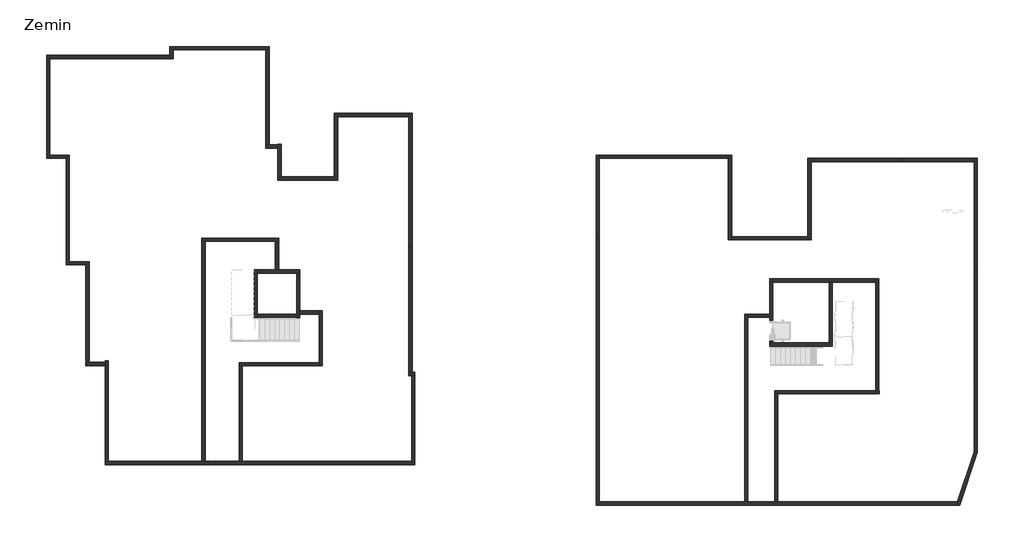
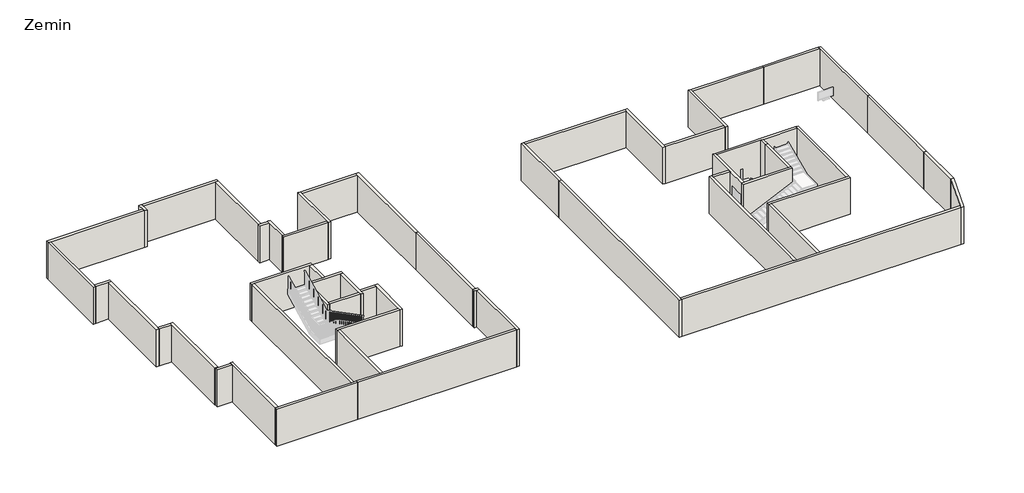
# One storey, part 1 of 2: 56 walls.
"""IFC4 building model written with IfcOpenShell, lengths in millimetres."""

from ifc_helpers import new_model, si_unit, origin, origin_with_axes, place, context, project, spatial, polyline, outline, extrude, faceted_brep, element, save

model = new_model("IFC4")

# Units and contexts
model_context = context("Model", 3, world=origin())
ifc_project = project(units=[si_unit("LENGTHUNIT", "METRE", prefix="MILLI")], contexts=[model_context])

# Site, building, storey
site = spatial("IfcSite", under=ifc_project)
building = spatial("IfcBuilding", under=site)
storey = spatial("IfcBuildingStorey", under=building, Name="Zemin", Elevation=0.0)

# Walls
placement = place(None, origin())
element("IfcWall", 1, ObjectType="Generic - 200mm", at=placement, inside=storey, context=model_context, shape_type="Brep", body=[
    faceted_brep([(25749.836337, 7619.475628, 0.0), (30068.3425199, 7619.475628, 0.0), (30068.3425199, 7619.475628, 3000.0), (25749.836337, 7619.475628, 3000.0), (25749.836337, 7819.475628, 0.0), (25749.836337, 7819.475628, 3000.0), (30068.3425199, 7819.475628, 3000.0), (30068.3425199, 7819.475628, 0.0), (30068.3425199, 7621.2707349, 3000.0)], [[[0, 1, 2, 3]], [[4, 5, 6, 7]], [[1, 0, 4, 7]], [[3, 2, 8, 6, 5]], [[0, 3, 5, 4]], [[2, 1, 7, 6, 8]]]),
])
element("IfcWall", 2, ObjectType="Generic - 200mm", at=placement, inside=storey, context=model_context, shape_type="Brep", body=[
    faceted_brep([(30068.3425199, 7819.475628, 0.0), (30068.3425199, 7619.475628, 0.0), (30068.3425199, 1319.475628, 0.0), (30068.3425199, 1319.475628, 3000.0), (30068.3425199, 7619.475628, 3000.0), (30068.3425199, 7819.475628, 3000.0), (30268.3425199, 7819.475628, 0.0), (30268.3425199, 7819.475628, 3000.0), (30268.3425199, 1319.475628, 3000.0), (30268.3425199, 1319.475628, 0.0), (30068.8612349, 1319.475628, 0.0), (30068.8612349, 1319.475628, 3000.0)], [[[0, 1, 2, 3, 4, 5]], [[6, 7, 8, 9]], [[2, 1, 0, 6, 9, 10]], [[3, 2, 10, 9, 8, 11]], [[5, 4, 3, 11, 8, 7]], [[0, 5, 7, 6]]]),
])
element("IfcWall", 3, ObjectType="Generic - 200mm", at=placement, inside=storey, context=model_context, shape_type="Brep", body=[
    faceted_brep([(30068.8612349, 1319.475628, 0.0), (30068.8612349, -6240.0098119, 0.0), (30068.8612349, -6240.0098119, 3000.0), (30068.8612349, 1319.475628, 3000.0), (30268.8612349, 1319.475628, 0.0), (30268.8612349, 1319.475628, 3000.0), (30268.8612349, -6240.0098119, 3000.0), (30268.8612349, -6240.0098119, 0.0), (30268.3425199, 1319.475628, 0.0), (30069.3799498, -6240.0098119, 0.0), (30069.3799498, -6240.0098119, 3000.0), (30268.3425199, 1319.475628, 3000.0)], [[[0, 1, 2, 3]], [[4, 5, 6, 7]], [[1, 0, 8, 4, 7, 9]], [[2, 1, 9, 7, 6, 10]], [[3, 2, 10, 6, 5, 11]], [[0, 3, 11, 5, 4, 8]]]),
])
element("IfcWall", 4, ObjectType="Generic - 200mm", at=placement, inside=storey, context=model_context, shape_type="Brep", body=[
    faceted_brep([(30069.3799498, -6240.0098119, 0.0), (30069.3799498, -9831.8731192, 0.0), (30069.3799498, -9831.8731192, 3000.0), (30069.3799498, -9830.0780123, 3000.0), (30069.3799498, -6240.0098119, 3000.0), (30269.3799498, -6240.0098119, 0.0), (30269.3799498, -6240.0098119, 3000.0), (30269.3799498, -9862.9162623, 3000.0), (30269.3799498, -9864.7113693, 3000.0), (30269.3799498, -9864.7113693, 0.0), (30268.8612349, -6240.0098119, 0.0), (30268.8612349, -6240.0098119, 3000.0)], [[[0, 1, 2, 3, 4]], [[5, 6, 7, 8, 9]], [[1, 0, 10, 5, 9]], [[4, 3, 2, 8, 7, 6, 11]], [[0, 4, 11, 6, 5, 10]], [[2, 1, 9, 8]]]),
])
element("IfcWall", 5, ObjectType="Generic - 200mm", at=placement, inside=storey, context=model_context, shape_type="Brep", body=[
    faceted_brep([(21549.836337, -3276.2808257, 0.0), (21349.836337, -3276.2808257, 0.0), (17970.6041014, -3276.2808257, 0.0), (17770.6041014, -3276.2808257, 0.0), (17770.6041014, -3276.2808257, 3000.0), (17970.6041014, -3276.2808257, 3000.0), (21349.836337, -3276.2808257, 3000.0), (21549.836337, -3276.2808257, 3000.0), (21549.836337, -3476.2808257, 0.0), (21549.836337, -3476.2808257, 3000.0), (17770.6041014, -3476.2808257, 3000.0), (17770.6041014, -3476.2808257, 0.0), (17770.6041014, -3474.4857187, 3000.0), (21549.836337, -3474.4857187, 3000.0)], [[[0, 1, 2, 3, 4, 5, 6, 7]], [[8, 9, 10, 11]], [[3, 2, 1, 0, 8, 11]], [[7, 6, 5, 4, 12, 10, 9, 13]], [[0, 7, 13, 9, 8]], [[4, 3, 11, 10, 12]]]),
])
element("IfcWall", 6, ObjectType="Generic - 200mm", at=placement, inside=storey, context=model_context, shape_type="Brep", body=[
    faceted_brep([(29055.3124022, -12836.6907835, 0.0), (18270.6041014, -12836.6907835, 0.0), (18070.6041014, -12836.6907835, 0.0), (16470.6041014, -12836.6907835, 0.0), (16270.6041014, -12836.6907835, 0.0), (7543.716007, -12836.6907835, 0.0), (7543.716007, -12836.6907835, 3000.0), (16270.6041014, -12836.6907835, 3000.0), (16470.6041014, -12836.6907835, 3000.0), (18070.6041014, -12836.6907835, 3000.0), (18270.6041014, -12836.6907835, 3000.0), (29055.3124022, -12836.6907835, 3000.0), (28987.8162902, -13036.6907835, 0.0), (28987.8162902, -13036.6907835, 3000.0), (7543.716007, -13036.6907835, 3000.0), (7543.716007, -13036.6907835, 0.0), (7543.716007, -13034.8956765, 3000.0)], [[[0, 1, 2, 3, 4, 5, 6, 7, 8, 9, 10, 11]], [[12, 13, 14, 15]], [[5, 4, 3, 2, 1, 0, 12, 15]], [[11, 10, 9, 8, 7, 6, 16, 14, 13]], [[0, 11, 13, 12]], [[6, 5, 15, 14, 16]]]),
])
element("IfcWall", 7, ObjectType="Generic - 200mm", at=placement, inside=storey, context=model_context, shape_type="Brep", body=[
    faceted_brep([(30069.3799498, -9831.8731192, 0.0), (29055.3124022, -12836.6907835, 0.0), (28987.8162902, -13036.6907835, 0.0), (28987.8162902, -13036.6907835, 3000.0), (29055.3124022, -12836.6907835, 3000.0), (30069.3799498, -9831.8731192, 3000.0), (30269.3799498, -9864.7113693, 0.0), (30269.3799498, -9864.7113693, 3000.0), (29198.8985612, -13036.6907835, 3000.0), (29198.8985612, -13036.6907835, 0.0)], [[[0, 1, 2, 3, 4, 5]], [[6, 7, 8, 9]], [[2, 1, 0, 6, 9]], [[5, 4, 3, 8, 7]], [[0, 5, 7, 6]], [[3, 2, 9, 8]]]),
])
element("IfcWall", 8, ObjectType="Generic - 200mm", at=placement, inside=storey, context=model_context, shape_type="Brep", body=[
    faceted_brep([(24363.3998354, -6140.0098119, 0.0), (24348.8612349, -6140.0098119, 0.0), (24148.8612349, -6140.0098119, 0.0), (18070.6041014, -6140.0098119, 0.0), (18070.6041014, -6140.0098119, 3000.0), (24148.8612349, -6140.0098119, 3000.0), (24348.8612349, -6140.0098119, 3000.0), (24363.3998354, -6140.0098119, 3000.0), (24363.3998354, -6340.0098119, 0.0), (24363.3998354, -6340.0098119, 3000.0), (18270.6041014, -6340.0098119, 3000.0), (18070.6041014, -6340.0098119, 3000.0), (18070.6041014, -6340.0098119, 0.0), (18270.6041014, -6340.0098119, 0.0)], [[[0, 1, 2, 3, 4, 5, 6, 7]], [[8, 9, 10, 11, 12, 13]], [[3, 2, 1, 0, 8, 13, 12]], [[7, 6, 5, 4, 11, 10, 9]], [[0, 7, 9, 8]], [[4, 3, 12, 11]]]),
])
element("IfcWall", 9, ObjectType="Generic - 200mm", at=placement, inside=storey, context=model_context, shape_type="Brep", body=[
    faceted_brep([(7343.716007, 3020.535295, 0.0), (7343.716007, -13036.6907835, 0.0), (7343.716007, -13036.6907835, 3000.0), (7343.716007, -13034.8956765, 3000.0), (7343.716007, 2920.535295, 3000.0), (7343.716007, 3020.535295, 3000.0), (7543.716007, 3020.535295, 0.0), (7543.716007, 3020.535295, 3000.0), (7543.716007, 2920.535295, 3000.0), (7543.716007, -12836.6907835, 3000.0), (7543.716007, -13034.8956765, 3000.0), (7543.716007, -13036.6907835, 3000.0), (7543.716007, -13036.6907835, 0.0), (7543.716007, -12836.6907835, 0.0)], [[[0, 1, 2, 3, 4, 5]], [[6, 7, 8, 9, 10, 11, 12, 13]], [[1, 0, 6, 13, 12]], [[5, 4, 3, 2, 11, 10, 9, 8, 7]], [[0, 5, 7, 6]], [[2, 1, 12, 11]]]),
])
element("IfcWall", 10, ObjectType="Generic - 200mm", at=placement, inside=storey, context=model_context, shape_type="Brep", body=[
    faceted_brep([(24348.8612349, -6140.0098119, 0.0), (24348.8612349, 579.475628, 0.0), (24348.8612349, 579.475628, 3000.0), (24348.8612349, -6140.0098119, 3000.0), (24148.8612349, -6140.0098119, 0.0), (24148.8612349, -6140.0098119, 3000.0), (24148.8612349, 379.475628, 3000.0), (24148.8612349, 579.475628, 3000.0), (24148.8612349, 579.475628, 0.0), (24148.8612349, 379.475628, 0.0)], [[[0, 1, 2, 3]], [[4, 5, 6, 7, 8, 9]], [[1, 0, 4, 9, 8]], [[3, 2, 7, 6, 5]], [[0, 3, 5, 4]], [[2, 1, 8, 7]]]),
])
element("IfcWall", 11, ObjectType="Generic - 200mm", at=placement, inside=storey, context=model_context, shape_type="Brep", body=[
    faceted_brep([(21349.836337, -200.524372, 0.0), (21349.836337, -3276.2808257, 0.0), (21349.836337, -3276.2808257, 3000.0), (21349.836337, -3274.4857187, 3000.0), (21349.836337, -200.524372, 3000.0), (21549.836337, -200.524372, 0.0), (21549.836337, -200.524372, 3000.0), (21549.836337, -3274.4857187, 3000.0), (21549.836337, -3276.2808257, 3000.0), (21549.836337, -3276.2808257, 0.0)], [[[0, 1, 2, 3, 4]], [[5, 6, 7, 8, 9]], [[1, 0, 5, 9]], [[4, 3, 2, 8, 7, 6]], [[0, 4, 6, 5]], [[2, 1, 9, 8]]]),
])
element("IfcWall", 12, ObjectType="Generic - 200mm", at=placement, inside=storey, context=model_context, shape_type="Brep", body=[
    faceted_brep([(17770.6041014, -3276.2808257, 3000.0), (17770.6041014, -3274.4857187, 3000.0), (17770.6041014, -3179.4925158, 3000.0), (17770.6041014, -1924.4857188, 3000.0), (17770.6041014, -1740.0098119, 3000.0), (17770.6041014, -1540.0098119, 3000.0), (17770.6041014, 579.475628, 3000.0), (17770.6041014, 579.475628, 0.0), (17770.6041014, -1540.0098119, 0.0), (17770.6041014, -1740.0098119, 0.0), (17770.6041014, -1926.2808257, 0.0), (17770.6041014, -1926.2808257, 2000.0), (17770.6041014, -3181.2876228, 2000.0), (17770.6041014, -3181.2876228, 0.0), (17770.6041014, -3276.2808257, 0.0), (17970.6041014, 579.475628, 3000.0), (17970.6041014, 379.475628, 3000.0), (17970.6041014, -1924.4857188, 3000.0), (17970.6041014, -3179.4925158, 3000.0), (17970.6041014, -3274.4857187, 3000.0), (17970.6041014, -3276.2808257, 3000.0), (17970.6041014, -3276.2808257, 0.0), (17970.6041014, -3181.2876228, 0.0), (17970.6041014, -3181.2876228, 2000.0), (17970.6041014, -1926.2808257, 2000.0), (17970.6041014, -1926.2808257, 0.0), (17970.6041014, 379.475628, 0.0), (17970.6041014, 579.475628, 0.0)], [[[0, 1, 2, 3, 4, 5, 6, 7, 8, 9, 10, 11, 12, 13, 14]], [[15, 16, 17, 18, 19, 20, 21, 22, 23, 24, 25, 26, 27]], [[21, 14, 13, 22]], [[7, 27, 26, 25, 10, 9, 8]], [[6, 5, 4, 3, 2, 1, 0, 20, 19, 18, 17, 16, 15]], [[0, 14, 21, 20]], [[12, 23, 22, 13]], [[24, 11, 10, 25]], [[11, 24, 23, 12]], [[27, 7, 6, 15]]]),
])
element("IfcWall", 13, ObjectType="Generic - 200mm", at=placement, inside=storey, context=model_context, shape_type="SweptSolid", body=[
    extrude(outline(polyline([(21549.836337, 379.475628), (21549.836337, -200.524372), (21349.836337, -200.524372), (21349.836337, 379.475628), (21549.836337, 379.475628)])), origin_with_axes(), (0.0, 0.0, 1.0), 3000.0),
])
element("IfcWall", 14, ObjectType="Generic - 200mm", at=placement, inside=storey, context=model_context, shape_type="Brep", body=[
    faceted_brep([(20268.8612349, 7619.475628, 0.0), (25749.836337, 7619.475628, 0.0), (25749.836337, 7619.475628, 3000.0), (20268.8612349, 7619.475628, 3000.0), (20268.8612349, 7819.475628, 0.0), (20268.8612349, 7819.475628, 3000.0), (25749.836337, 7819.475628, 3000.0), (25749.836337, 7819.475628, 0.0), (20268.8612349, 7621.2707349, 3000.0)], [[[0, 1, 2, 3]], [[4, 5, 6, 7]], [[1, 0, 4, 7]], [[2, 1, 7, 6]], [[3, 2, 6, 5, 8]], [[0, 3, 8, 5, 4]]]),
])
element("IfcWall", 15, ObjectType="Generic - 200mm", at=placement, inside=storey, context=model_context, shape_type="Brep", body=[
    faceted_brep([(16470.6041014, -12836.6907835, 0.0), (16470.6041014, -1740.0098119, 0.0), (16470.6041014, -1540.0098119, 0.0), (16470.6041014, -1540.0098119, 3000.0), (16470.6041014, -1740.0098119, 3000.0), (16470.6041014, -12836.6907835, 3000.0), (16270.6041014, -12836.6907835, 0.0), (16270.6041014, -12836.6907835, 3000.0), (16270.6041014, -1540.0098119, 3000.0), (16270.6041014, -1540.0098119, 0.0)], [[[0, 1, 2, 3, 4, 5]], [[6, 7, 8, 9]], [[2, 1, 0, 6, 9]], [[5, 4, 3, 8, 7]], [[3, 2, 9, 8]], [[0, 5, 7, 6]]]),
])
element("IfcWall", 16, ObjectType="Generic - 200mm", at=placement, inside=storey, context=model_context, shape_type="Brep", body=[
    faceted_brep([(20068.8612349, 7819.475628, 0.0), (20068.8612349, 3119.475628, 0.0), (20068.8612349, 2919.475628, 0.0), (20068.8612349, 2919.475628, 3000.0), (20068.8612349, 2921.2707349, 3000.0), (20068.8612349, 3119.475628, 3000.0), (20068.8612349, 7819.475628, 3000.0), (20268.8612349, 7819.475628, 0.0), (20268.8612349, 7819.475628, 3000.0), (20268.8612349, 7619.475628, 3000.0), (20268.8612349, 2921.2707349, 3000.0), (20268.8612349, 2919.475628, 3000.0), (20268.8612349, 2919.475628, 0.0), (20268.8612349, 7619.475628, 0.0)], [[[0, 1, 2, 3, 4, 5, 6]], [[7, 8, 9, 10, 11, 12, 13]], [[2, 1, 0, 7, 13, 12]], [[6, 5, 4, 3, 11, 10, 9, 8]], [[0, 6, 8, 7]], [[3, 2, 12, 11]]]),
])
element("IfcWall", 17, ObjectType="Generic - 200mm", at=placement, inside=storey, context=model_context, shape_type="Brep", body=[
    faceted_brep([(24148.8612349, 579.475628, 0.0), (17970.6041014, 579.475628, 0.0), (17970.6041014, 579.475628, 3000.0), (24148.8612349, 579.475628, 3000.0), (24148.8612349, 379.475628, 0.0), (24148.8612349, 379.475628, 3000.0), (21549.836337, 379.475628, 3000.0), (21349.836337, 379.475628, 3000.0), (17970.6041014, 379.475628, 3000.0), (17970.6041014, 379.475628, 0.0), (21349.836337, 379.475628, 0.0), (21549.836337, 379.475628, 0.0)], [[[0, 1, 2, 3]], [[4, 5, 6, 7, 8, 9, 10, 11]], [[1, 0, 4, 11, 10, 9]], [[3, 2, 8, 7, 6, 5]], [[2, 1, 9, 8]], [[0, 3, 5, 4]]]),
])
element("IfcWall", 18, ObjectType="Generic - 200mm", at=placement, inside=storey, context=model_context, shape_type="Brep", body=[
    faceted_brep([(-3749.8304233, -5256.848891, 0.0), (-3749.8304233, -10389.1627129, 0.0), (-3749.8304233, -10589.1627129, 0.0), (-3749.8304233, -10589.1627129, 3000.0), (-3749.8304233, -10587.367606, 3000.0), (-3749.8304233, -10389.1627129, 3000.0), (-3749.8304233, -5256.848891, 3000.0), (-3549.8304233, -5256.848891, 0.0), (-3549.8304233, -5256.848891, 3000.0), (-3549.8304233, -10587.367606, 3000.0), (-3549.8304233, -10589.1627129, 3000.0), (-3549.8304233, -10589.1627129, 0.0)], [[[0, 1, 2, 3, 4, 5, 6]], [[7, 8, 9, 10, 11]], [[2, 1, 0, 7, 11]], [[6, 5, 4, 3, 10, 9, 8]], [[3, 2, 11, 10]], [[0, 6, 8, 7]]]),
])
element("IfcWall", 19, ObjectType="Generic - 200mm", at=placement, inside=storey, context=model_context, shape_type="Brep", body=[
    faceted_brep([(-3749.8304233, -10389.1627129, 0.0), (-13926.101437, -10389.1627129, 0.0), (-14126.101437, -10389.1627129, 0.0), (-15974.8304233, -10389.1627129, 0.0), (-15974.8304233, -10389.1627129, 3000.0), (-14126.101437, -10389.1627129, 3000.0), (-13926.101437, -10389.1627129, 3000.0), (-3749.8304233, -10389.1627129, 3000.0), (-3749.8304233, -10589.1627129, 0.0), (-3749.8304233, -10589.1627129, 3000.0), (-15974.8304233, -10589.1627129, 3000.0), (-15974.8304233, -10589.1627129, 0.0), (-15974.8304233, -10389.6814279, 0.0), (-15974.8304233, -10587.367606, 3000.0), (-15974.8304233, -10389.6814279, 3000.0), (-3749.8304233, -10587.367606, 3000.0)], [[[0, 1, 2, 3, 4, 5, 6, 7]], [[8, 9, 10, 11]], [[3, 2, 1, 0, 8, 11, 12]], [[4, 3, 12, 11, 10, 13, 14]], [[7, 6, 5, 4, 14, 13, 10, 9, 15]], [[0, 7, 15, 9, 8]]]),
])
element("IfcWall", 20, ObjectType="Generic - 200mm", at=placement, inside=storey, context=model_context, shape_type="Brep", body=[
    faceted_brep([(-15974.8304233, -10389.6814279, 0.0), (-16173.9741722, -10389.6814279, 0.0), (-16373.9741722, -10389.6814279, 0.0), (-21985.6447259, -10389.6814279, 0.0), (-22185.6447259, -10389.6814279, 0.0), (-22185.6447259, -10389.6814279, 3000.0), (-21985.6447259, -10389.6814279, 3000.0), (-16373.9741722, -10389.6814279, 3000.0), (-16173.9741722, -10389.6814279, 3000.0), (-15974.8304233, -10389.6814279, 3000.0), (-15974.8304233, -10589.6814279, 0.0), (-15974.8304233, -10589.6814279, 3000.0), (-22185.6447259, -10589.6814279, 3000.0), (-22185.6447259, -10589.6814279, 0.0), (-15974.8304233, -10589.1627129, 0.0), (-22185.6447259, -10587.886321, 3000.0), (-15974.8304233, -10589.1627129, 3000.0), (-15974.8304233, -10587.886321, 3000.0)], [[[0, 1, 2, 3, 4, 5, 6, 7, 8, 9]], [[10, 11, 12, 13]], [[4, 3, 2, 1, 0, 14, 10, 13]], [[9, 8, 7, 6, 5, 15, 12, 11, 16, 17]], [[0, 9, 17, 16, 11, 10, 14]], [[5, 4, 13, 12, 15]]]),
])
element("IfcWall", 21, ObjectType="Generic - 200mm", at=placement, inside=storey, context=model_context, shape_type="Brep", body=[
    faceted_brep([(-13026.101437, -1740.1378151, 0.0), (-13026.101437, -1540.1378151, 0.0), (-13026.101437, 920.8372871, 0.0), (-13026.101437, 1120.8372871, 0.0), (-13026.101437, 1120.8372871, 3000.0), (-13026.101437, 920.8372871, 3000.0), (-13026.101437, -1540.1378151, 3000.0), (-13026.101437, -1738.3427081, 3000.0), (-13026.101437, -1740.1378151, 3000.0), (-13226.101437, -1740.1378151, 0.0), (-13226.101437, -1740.1378151, 3000.0), (-13226.101437, -1738.3427081, 3000.0), (-13226.101437, 1120.8372871, 3000.0), (-13226.101437, 1120.8372871, 0.0)], [[[0, 1, 2, 3, 4, 5, 6, 7, 8]], [[9, 10, 11, 12, 13]], [[3, 2, 1, 0, 9, 13]], [[8, 7, 6, 5, 4, 12, 11, 10]], [[0, 8, 10, 9]], [[4, 3, 13, 12]]]),
])
element("IfcWall", 22, ObjectType="Generic - 200mm", at=placement, inside=storey, context=model_context, shape_type="Brep", body=[
    faceted_brep([(-23146.5113948, -4345.3648645, 0.0), (-23146.5113948, 1614.6351355, 0.0), (-23146.5113948, 1614.6351355, 3000.0), (-23146.5113948, -4345.3648645, 3000.0), (-23346.5113948, -4345.3648645, 0.0), (-23346.5113948, -4345.3648645, 3000.0), (-23346.5113948, 1414.6351355, 3000.0), (-23346.5113948, 1614.6351355, 3000.0), (-23346.5113948, 1614.6351355, 0.0), (-23346.5113948, 1414.6351355, 0.0)], [[[0, 1, 2, 3]], [[4, 5, 6, 7, 8, 9]], [[1, 0, 4, 9, 8]], [[3, 2, 7, 6, 5]], [[0, 3, 5, 4]], [[2, 1, 8, 7]]]),
])
element("IfcWall", 23, ObjectType="Generic - 200mm", at=placement, inside=storey, context=model_context, shape_type="SweptSolid", body=[
    extrude(outline(polyline([(-16173.9741722, 2820.8372871), (-16173.9741722, -10389.6814279), (-16373.9741722, -10389.6814279), (-16373.9741722, 2820.8372871), (-16173.9741722, 2820.8372871)])), origin_with_axes(), (0.0, 0.0, 1.0), 3000.0),
])
element("IfcWall", 24, ObjectType="Generic - 200mm", at=placement, inside=storey, context=model_context, shape_type="Brep", body=[
    faceted_brep([(-14126.101437, -4659.1627129, 0.0), (-13926.101437, -4659.1627129, 0.0), (-9310.3884323, -4659.1627129, 0.0), (-9310.3884323, -4659.1627129, 3000.0), (-13926.101437, -4659.1627129, 3000.0), (-14126.101437, -4659.1627129, 3000.0), (-14126.101437, -4459.1627129, 0.0), (-14126.101437, -4459.1627129, 3000.0), (-9310.3884323, -4459.1627129, 3000.0), (-9310.3884323, -4459.1627129, 0.0), (-9310.3884323, -4657.367606, 3000.0)], [[[0, 1, 2, 3, 4, 5]], [[6, 7, 8, 9]], [[2, 1, 0, 6, 9]], [[5, 4, 3, 10, 8, 7]], [[3, 2, 9, 8, 10]], [[0, 5, 7, 6]]]),
])
element("IfcWall", 25, ObjectType="Generic - 200mm", at=placement, inside=storey, context=model_context, shape_type="Brep", body=[
    faceted_brep([(-10669.8304233, -1540.1378151, 0.0), (-13026.101437, -1540.1378151, 0.0), (-13026.101437, -1540.1378151, 3000.0), (-10669.8304233, -1540.1378151, 3000.0), (-10669.8304233, -1740.1378151, 0.0), (-10669.8304233, -1740.1378151, 3000.0), (-13026.101437, -1740.1378151, 3000.0), (-13026.101437, -1740.1378151, 0.0), (-13026.101437, -1738.3427081, 3000.0)], [[[0, 1, 2, 3]], [[4, 5, 6, 7]], [[1, 0, 4, 7]], [[3, 2, 8, 6, 5]], [[2, 1, 7, 6, 8]], [[0, 3, 5, 4]]]),
])
element("IfcWall", 26, ObjectType="Generic - 200mm", at=placement, inside=storey, context=model_context, shape_type="Brep", body=[
    faceted_brep([(-10469.8304233, 1120.8372871, 0.0), (-11746.101437, 1120.8372871, 0.0), (-11946.101437, 1120.8372871, 0.0), (-13026.101437, 1120.8372871, 0.0), (-13026.101437, 1120.8372871, 3000.0), (-11946.101437, 1120.8372871, 3000.0), (-11746.101437, 1120.8372871, 3000.0), (-10469.8304233, 1120.8372871, 3000.0), (-10469.8304233, 920.8372871, 0.0), (-10469.8304233, 920.8372871, 3000.0), (-10669.8304233, 920.8372871, 3000.0), (-13026.101437, 920.8372871, 3000.0), (-13026.101437, 920.8372871, 0.0), (-10669.8304233, 920.8372871, 0.0), (-13026.101437, 922.632394, 3000.0), (-10469.8304233, 922.632394, 3000.0)], [[[0, 1, 2, 3, 4, 5, 6, 7]], [[8, 9, 10, 11, 12, 13]], [[3, 2, 1, 0, 8, 13, 12]], [[7, 6, 5, 4, 14, 11, 10, 9, 15]], [[0, 7, 15, 9, 8]], [[4, 3, 12, 11, 14]]]),
])
element("IfcWall", 27, ObjectType="Generic - 200mm", at=placement, inside=storey, context=model_context, shape_type="Brep", body=[
    faceted_brep([(-10469.8304233, -1779.1627129, 0.0), (-10469.8304233, -1540.1378151, 0.0), (-10469.8304233, -1340.1378151, 0.0), (-10469.8304233, 920.8372871, 0.0), (-10469.8304233, 920.8372871, 3000.0), (-10469.8304233, -1340.1378151, 3000.0), (-10469.8304233, -1540.1378151, 3000.0), (-10469.8304233, -1777.367606, 3000.0), (-10469.8304233, -1779.1627129, 3000.0), (-10669.8304233, -1779.1627129, 0.0), (-10669.8304233, -1779.1627129, 3000.0), (-10669.8304233, -1777.367606, 3000.0), (-10669.8304233, -1740.1378151, 3000.0), (-10669.8304233, -1540.1378151, 3000.0), (-10669.8304233, 920.8372871, 3000.0), (-10669.8304233, 920.8372871, 0.0), (-10669.8304233, -1540.1378151, 0.0), (-10669.8304233, -1740.1378151, 0.0)], [[[0, 1, 2, 3, 4, 5, 6, 7, 8]], [[9, 10, 11, 12, 13, 14, 15, 16, 17]], [[3, 2, 1, 0, 9, 17, 16, 15]], [[8, 7, 6, 5, 4, 14, 13, 12, 11, 10]], [[0, 8, 10, 9]], [[4, 3, 15, 14]]]),
])
element("IfcWall", 28, ObjectType="Generic - 200mm", at=placement, inside=storey, context=model_context, shape_type="Brep", body=[
    faceted_brep([(-12326.101437, 14540.8372871, 0.0), (-18089.8304233, 14540.8372871, 0.0), (-18089.8304233, 14540.8372871, 3000.0), (-12326.101437, 14540.8372871, 3000.0), (-12326.101437, 14340.8372871, 0.0), (-12326.101437, 14340.8372871, 3000.0), (-12526.101437, 14340.8372871, 3000.0), (-18089.8304233, 14340.8372871, 3000.0), (-18089.8304233, 14340.8372871, 0.0), (-12526.101437, 14340.8372871, 0.0), (-18089.8304233, 14342.632394, 3000.0), (-12326.101437, 14342.632394, 3000.0)], [[[0, 1, 2, 3]], [[4, 5, 6, 7, 8, 9]], [[1, 0, 4, 9, 8]], [[3, 2, 10, 7, 6, 5, 11]], [[2, 1, 8, 7, 10]], [[0, 3, 11, 5, 4]]]),
])
element("IfcWall", 29, ObjectType="Generic - 200mm", at=placement, inside=storey, context=model_context, shape_type="Brep", body=[
    faceted_brep([(-25701.4369496, 13812.8400285, 0.0), (-25701.4369496, 7812.8400285, 0.0), (-25701.4369496, 7812.8400285, 3000.0), (-25701.4369496, 7814.6351355, 3000.0), (-25701.4369496, 13812.8400285, 3000.0), (-25501.4369496, 13812.8400285, 0.0), (-25501.4369496, 13812.8400285, 3000.0), (-25501.4369496, 8012.8400285, 3000.0), (-25501.4369496, 7814.6351355, 3000.0), (-25501.4369496, 7812.8400285, 3000.0), (-25501.4369496, 7812.8400285, 0.0), (-25501.4369496, 8012.8400285, 0.0)], [[[0, 1, 2, 3, 4]], [[5, 6, 7, 8, 9, 10, 11]], [[1, 0, 5, 11, 10]], [[4, 3, 2, 9, 8, 7, 6]], [[2, 1, 10, 9]], [[0, 4, 6, 5]]]),
])
element("IfcWall", 30, ObjectType="Generic - 200mm", at=placement, inside=storey, context=model_context, shape_type="Brep", body=[
    faceted_brep([(-25501.4369496, 7812.8400285, 0.0), (-24523.9741722, 7812.8400285, 0.0), (-24323.9741722, 7812.8400285, 0.0), (-24323.9741722, 7812.8400285, 3000.0), (-24523.9741722, 7812.8400285, 3000.0), (-25501.4369496, 7812.8400285, 3000.0), (-25501.4369496, 8012.8400285, 0.0), (-25501.4369496, 8012.8400285, 3000.0), (-24323.9741722, 8012.8400285, 3000.0), (-24323.9741722, 8012.8400285, 0.0), (-25501.4369496, 7814.6351355, 3000.0)], [[[0, 1, 2, 3, 4, 5]], [[6, 7, 8, 9]], [[2, 1, 0, 6, 9]], [[5, 4, 3, 8, 7, 10]], [[0, 5, 10, 7, 6]], [[3, 2, 9, 8]]]),
])
element("IfcWall", 31, ObjectType="Generic - 200mm", at=placement, inside=storey, context=model_context, shape_type="Brep", body=[
    faceted_brep([(-18289.8304233, 14012.8400285, 0.0), (-25701.4369496, 14012.8400285, 0.0), (-25701.4369496, 14012.8400285, 3000.0), (-18289.8304233, 14012.8400285, 3000.0), (-18289.8304233, 13812.8400285, 0.0), (-18289.8304233, 13812.8400285, 3000.0), (-25501.4369496, 13812.8400285, 3000.0), (-25701.4369496, 13812.8400285, 3000.0), (-25701.4369496, 13812.8400285, 0.0), (-25501.4369496, 13812.8400285, 0.0), (-25701.4369496, 13814.6351355, 3000.0), (-18289.8304233, 13814.6351355, 3000.0)], [[[0, 1, 2, 3]], [[4, 5, 6, 7, 8, 9]], [[1, 0, 4, 9, 8]], [[3, 2, 10, 7, 6, 5, 11]], [[2, 1, 8, 7, 10]], [[0, 3, 11, 5, 4]]]),
])
element("IfcWall", 32, ObjectType="Generic - 200mm", at=placement, inside=storey, context=model_context, shape_type="Brep", body=[
    faceted_brep([(-24523.9741722, 7812.8400285, 0.0), (-24523.9741722, 1414.6351355, 0.0), (-24523.9741722, 1414.6351355, 3000.0), (-24523.9741722, 7812.8400285, 3000.0), (-24323.9741722, 7812.8400285, 0.0), (-24323.9741722, 7812.8400285, 3000.0), (-24323.9741722, 1614.6351355, 3000.0), (-24323.9741722, 1414.6351355, 3000.0), (-24323.9741722, 1414.6351355, 0.0), (-24323.9741722, 1614.6351355, 0.0)], [[[0, 1, 2, 3]], [[4, 5, 6, 7, 8, 9]], [[1, 0, 4, 9, 8]], [[3, 2, 7, 6, 5]], [[0, 3, 5, 4]], [[2, 1, 8, 7]]]),
])
element("IfcWall", 33, ObjectType="Generic - 200mm", at=placement, inside=storey, context=model_context, shape_type="Brep", body=[
    faceted_brep([(-21985.6447259, -10389.6814279, 0.0), (-21985.6447259, -4345.3648645, 0.0), (-21985.6447259, -4345.3648645, 3000.0), (-21985.6447259, -4445.3648645, 3000.0), (-21985.6447259, -10387.886321, 3000.0), (-21985.6447259, -10389.6814279, 3000.0), (-22185.6447259, -10389.6814279, 0.0), (-22185.6447259, -10389.6814279, 3000.0), (-22185.6447259, -10387.886321, 3000.0), (-22185.6447259, -4645.3648645, 3000.0), (-22185.6447259, -4445.3648645, 3000.0), (-22185.6447259, -4345.3648645, 3000.0), (-22185.6447259, -4345.3648645, 0.0), (-22185.6447259, -4445.3648645, 0.0), (-22185.6447259, -4645.3648645, 0.0)], [[[0, 1, 2, 3, 4, 5]], [[6, 7, 8, 9, 10, 11, 12, 13, 14]], [[1, 0, 6, 14, 13, 12]], [[2, 1, 12, 11]], [[5, 4, 3, 2, 11, 10, 9, 8, 7]], [[0, 5, 7, 6]]]),
])
element("IfcWall", 34, ObjectType="Generic - 200mm", at=placement, inside=storey, context=model_context, shape_type="Brep", body=[
    faceted_brep([(-8390.3449834, 6700.8372871, 0.0), (-11586.101437, 6700.8372871, 0.0), (-11786.101437, 6700.8372871, 0.0), (-11790.3449834, 6700.8372871, 0.0), (-11790.3449834, 6700.8372871, 3000.0), (-11786.101437, 6700.8372871, 3000.0), (-11586.101437, 6700.8372871, 3000.0), (-8390.3449834, 6700.8372871, 3000.0), (-8390.3449834, 6500.8372871, 0.0), (-8390.3449834, 6500.8372871, 3000.0), (-11790.3449834, 6500.8372871, 3000.0), (-11790.3449834, 6500.8372871, 0.0), (-8390.3449834, 6502.632394, 3000.0)], [[[0, 1, 2, 3, 4, 5, 6, 7]], [[8, 9, 10, 11]], [[3, 2, 1, 0, 8, 11]], [[4, 3, 11, 10]], [[7, 6, 5, 4, 10, 9, 12]], [[0, 7, 12, 9, 8]]]),
])
element("IfcWall", 35, ObjectType="Generic - 200mm", at=placement, inside=storey, context=model_context, shape_type="Brep", body=[
    faceted_brep([(-16373.9741722, 2820.8372871, 0.0), (-16173.9741722, 2820.8372871, 0.0), (-11946.101437, 2820.8372871, 0.0), (-11746.101437, 2820.8372871, 0.0), (-11746.101437, 2820.8372871, 3000.0), (-11946.101437, 2820.8372871, 3000.0), (-16173.9741722, 2820.8372871, 3000.0), (-16373.9741722, 2820.8372871, 3000.0), (-16373.9741722, 3020.8372871, 0.0), (-16373.9741722, 3020.8372871, 3000.0), (-11746.101437, 3020.8372871, 3000.0), (-11746.101437, 3020.8372871, 0.0)], [[[0, 1, 2, 3, 4, 5, 6, 7]], [[8, 9, 10, 11]], [[3, 2, 1, 0, 8, 11]], [[7, 6, 5, 4, 10, 9]], [[0, 7, 9, 8]], [[4, 3, 11, 10]]]),
])
element("IfcWall", 36, ObjectType="Generic - 200mm", at=placement, inside=storey, context=model_context, shape_type="Brep", body=[
    faceted_brep([(-3920.3449834, 2560.8372871, 0.0), (-3920.3449834, -5056.848891, 0.0), (-3920.3449834, -5056.848891, 3000.0), (-3920.3449834, -4956.848891, 3000.0), (-3920.3449834, 2560.8372871, 3000.0), (-3720.3449834, 2560.8372871, 0.0), (-3720.3449834, 2560.8372871, 3000.0), (-3720.3449834, -4956.848891, 3000.0), (-3720.3449834, -5056.848891, 3000.0), (-3720.3449834, -5056.848891, 0.0), (-3725.3449834, 2560.8372871, 0.0), (-3725.3449834, 2560.8372871, 3000.0)], [[[0, 1, 2, 3, 4]], [[5, 6, 7, 8, 9]], [[1, 0, 10, 5, 9]], [[4, 3, 2, 8, 7, 6, 11]], [[0, 4, 11, 6, 5, 10]], [[2, 1, 9, 8]]]),
])
element("IfcWall", 37, ObjectType="Generic - 200mm", at=placement, inside=storey, context=model_context, shape_type="Brep", body=[
    faceted_brep([(-9310.3884323, -1340.1378151, 0.0), (-9310.3884323, -1540.1378151, 0.0), (-9310.3884323, -4459.1627129, 0.0), (-9310.3884323, -4659.1627129, 0.0), (-9310.3884323, -4659.1627129, 3000.0), (-9310.3884323, -4657.367606, 3000.0), (-9310.3884323, -4459.1627129, 3000.0), (-9310.3884323, -1540.1378151, 3000.0), (-9310.3884323, -1340.1378151, 3000.0), (-9110.3884323, -1340.1378151, 0.0), (-9110.3884323, -1340.1378151, 3000.0), (-9110.3884323, -4657.367606, 3000.0), (-9110.3884323, -4659.1627129, 3000.0), (-9110.3884323, -4659.1627129, 0.0)], [[[0, 1, 2, 3, 4, 5, 6, 7, 8]], [[9, 10, 11, 12, 13]], [[3, 2, 1, 0, 9, 13]], [[8, 7, 6, 5, 4, 12, 11, 10]], [[0, 8, 10, 9]], [[4, 3, 13, 12]]]),
])
element("IfcWall", 38, ObjectType="Generic - 200mm", at=placement, inside=storey, context=model_context, shape_type="Brep", body=[
    faceted_brep([(-3925.3449834, 10520.8372871, 0.0), (-3925.3449834, 10320.8372871, 0.0), (-3925.3449834, 2560.8372871, 0.0), (-3925.3449834, 2560.8372871, 3000.0), (-3925.3449834, 10320.8372871, 3000.0), (-3925.3449834, 10520.8372871, 3000.0), (-3725.3449834, 10520.8372871, 0.0), (-3725.3449834, 10520.8372871, 3000.0), (-3725.3449834, 2560.8372871, 3000.0), (-3725.3449834, 2560.8372871, 0.0), (-3920.3449834, 2560.8372871, 0.0), (-3920.3449834, 2560.8372871, 3000.0)], [[[0, 1, 2, 3, 4, 5]], [[6, 7, 8, 9]], [[2, 1, 0, 6, 9, 10]], [[3, 2, 10, 9, 8, 11]], [[5, 4, 3, 11, 8, 7]], [[0, 5, 7, 6]]]),
])
element("IfcWall", 39, ObjectType="Generic - 200mm", at=placement, inside=storey, context=model_context, shape_type="Brep", body=[
    faceted_brep([(15488.8612349, 2919.475628, 0.0), (20068.8612349, 2919.475628, 0.0), (20068.8612349, 2919.475628, 3000.0), (15488.8612349, 2919.475628, 3000.0), (15488.8612349, 3119.475628, 0.0), (15488.8612349, 3119.475628, 3000.0), (20068.8612349, 3119.475628, 3000.0), (20068.8612349, 3119.475628, 0.0), (20068.8612349, 2921.2707349, 3000.0)], [[[0, 1, 2, 3]], [[4, 5, 6, 7]], [[1, 0, 4, 7]], [[3, 2, 8, 6, 5]], [[2, 1, 7, 6, 8]], [[0, 3, 5, 4]]]),
])
element("IfcWall", 40, ObjectType="Generic - 200mm", at=placement, inside=storey, context=model_context, shape_type="Brep", body=[
    faceted_brep([(7543.716007, 3020.535295, 0.0), (7543.716007, 7819.475628, 0.0), (7543.716007, 8019.475628, 0.0), (7543.716007, 8019.475628, 3000.0), (7543.716007, 7819.475628, 3000.0), (7543.716007, 3120.535295, 3000.0), (7543.716007, 3020.535295, 3000.0), (7343.716007, 3020.535295, 0.0), (7343.716007, 3020.535295, 3000.0), (7343.716007, 3120.535295, 3000.0), (7343.716007, 8019.475628, 3000.0), (7343.716007, 8019.475628, 0.0)], [[[0, 1, 2, 3, 4, 5, 6]], [[7, 8, 9, 10, 11]], [[2, 1, 0, 7, 11]], [[6, 5, 4, 3, 10, 9, 8]], [[0, 6, 8, 7]], [[3, 2, 11, 10]]]),
])
element("IfcWall", 41, ObjectType="Generic - 200mm", at=placement, inside=storey, context=model_context, shape_type="Brep", body=[
    faceted_brep([(15488.8612349, 2919.475628, 0.0), (15488.8612349, 3119.475628, 0.0), (15488.8612349, 8019.475628, 0.0), (15488.8612349, 8019.475628, 3000.0), (15488.8612349, 3119.475628, 3000.0), (15488.8612349, 2920.535295, 3000.0), (15488.8612349, 2919.475628, 3000.0), (15288.8612349, 2919.475628, 0.0), (15288.8612349, 2919.475628, 3000.0), (15288.8612349, 2920.535295, 3000.0), (15288.8612349, 7819.475628, 3000.0), (15288.8612349, 8019.475628, 3000.0), (15288.8612349, 8019.475628, 0.0), (15288.8612349, 7819.475628, 0.0)], [[[0, 1, 2, 3, 4, 5, 6]], [[7, 8, 9, 10, 11, 12, 13]], [[2, 1, 0, 7, 13, 12]], [[6, 5, 4, 3, 11, 10, 9, 8]], [[3, 2, 12, 11]], [[0, 6, 8, 7]]]),
])
element("IfcWall", 42, ObjectType="Generic - 200mm", at=placement, inside=storey, context=model_context, shape_type="Brep", body=[
    faceted_brep([(15288.8612349, 8019.475628, 0.0), (7543.716007, 8019.475628, 0.0), (7543.716007, 8019.475628, 3000.0), (15288.8612349, 8019.475628, 3000.0), (15288.8612349, 7819.475628, 0.0), (15288.8612349, 7819.475628, 3000.0), (7543.716007, 7819.475628, 3000.0), (7543.716007, 7819.475628, 0.0), (7543.716007, 7821.2707349, 3000.0), (15288.8612349, 7821.2707349, 3000.0)], [[[0, 1, 2, 3]], [[4, 5, 6, 7]], [[1, 0, 4, 7]], [[3, 2, 8, 6, 5, 9]], [[0, 3, 9, 5, 4]], [[2, 1, 7, 6, 8]]]),
])
element("IfcWall", 43, ObjectType="Generic - 200mm", at=placement, inside=storey, context=model_context, shape_type="Brep", body=[
    faceted_brep([(-12526.101437, 14340.8372871, 0.0), (-12526.101437, 8640.8372871, 0.0), (-12526.101437, 8640.8372871, 3000.0), (-12526.101437, 8642.632394, 3000.0), (-12526.101437, 14340.8372871, 3000.0), (-12326.101437, 14340.8372871, 0.0), (-12326.101437, 14340.8372871, 3000.0), (-12326.101437, 8642.632394, 3000.0), (-12326.101437, 8640.8372871, 3000.0), (-12326.101437, 8640.8372871, 0.0)], [[[0, 1, 2, 3, 4]], [[5, 6, 7, 8, 9]], [[1, 0, 5, 9]], [[4, 3, 2, 8, 7, 6]], [[0, 4, 6, 5]], [[2, 1, 9, 8]]]),
])
element("IfcWall", 44, ObjectType="Generic - 200mm", at=placement, inside=storey, context=model_context, shape_type="Brep", body=[
    faceted_brep([(-11786.101437, 8640.8372871, 0.0), (-12326.101437, 8640.8372871, 0.0), (-12526.101437, 8640.8372871, 0.0), (-12526.101437, 8640.8372871, 3000.0), (-12326.101437, 8640.8372871, 3000.0), (-11786.101437, 8640.8372871, 3000.0), (-11786.101437, 8440.8372871, 0.0), (-11786.101437, 8440.8372871, 3000.0), (-12526.101437, 8440.8372871, 3000.0), (-12526.101437, 8440.8372871, 0.0)], [[[0, 1, 2, 3, 4, 5]], [[6, 7, 8, 9]], [[2, 1, 0, 6, 9]], [[5, 4, 3, 8, 7]], [[0, 5, 7, 6]], [[3, 2, 9, 8]]]),
])
element("IfcWall", 45, ObjectType="Generic - 200mm", at=placement, inside=storey, context=model_context, shape_type="Brep", body=[
    faceted_brep([(-8190.3449834, 6500.8372871, 0.0), (-8190.3449834, 10320.8372871, 0.0), (-8190.3449834, 10520.8372871, 0.0), (-8190.3449834, 10520.8372871, 3000.0), (-8190.3449834, 10320.8372871, 3000.0), (-8190.3449834, 6502.632394, 3000.0), (-8190.3449834, 6500.8372871, 3000.0), (-8390.3449834, 6500.8372871, 0.0), (-8390.3449834, 6500.8372871, 3000.0), (-8390.3449834, 6502.632394, 3000.0), (-8390.3449834, 6700.8372871, 3000.0), (-8390.3449834, 10520.8372871, 3000.0), (-8390.3449834, 10520.8372871, 0.0), (-8390.3449834, 6700.8372871, 0.0)], [[[0, 1, 2, 3, 4, 5, 6]], [[7, 8, 9, 10, 11, 12, 13]], [[2, 1, 0, 7, 13, 12]], [[6, 5, 4, 3, 11, 10, 9, 8]], [[3, 2, 12, 11]], [[0, 6, 8, 7]]]),
])
element("IfcWall", 46, ObjectType="Generic - 200mm", at=placement, inside=storey, context=model_context, shape_type="Brep", body=[
    faceted_brep([(-8190.3449834, 10320.8372871, 0.0), (-3925.3449834, 10320.8372871, 0.0), (-3925.3449834, 10320.8372871, 3000.0), (-8190.3449834, 10320.8372871, 3000.0), (-8190.3449834, 10520.8372871, 0.0), (-8190.3449834, 10520.8372871, 3000.0), (-3925.3449834, 10520.8372871, 3000.0), (-3925.3449834, 10520.8372871, 0.0), (-3925.3449834, 10322.632394, 3000.0), (-8190.3449834, 10322.632394, 3000.0)], [[[0, 1, 2, 3]], [[4, 5, 6, 7]], [[1, 0, 4, 7]], [[3, 2, 8, 6, 5, 9]], [[0, 3, 9, 5, 4]], [[2, 1, 7, 6, 8]]]),
])
element("IfcWall", 47, ObjectType="Generic - 200mm", at=placement, inside=storey, context=model_context, shape_type="Brep", body=[
    faceted_brep([(-9310.3884323, -1340.1378151, 0.0), (-10469.8304233, -1340.1378151, 0.0), (-10469.8304233, -1340.1378151, 3000.0), (-9310.3884323, -1340.1378151, 3000.0), (-9310.3884323, -1540.1378151, 0.0), (-9310.3884323, -1540.1378151, 3000.0), (-10469.8304233, -1540.1378151, 3000.0), (-10469.8304233, -1540.1378151, 0.0), (-9310.3884323, -1538.3427081, 3000.0)], [[[0, 1, 2, 3]], [[4, 5, 6, 7]], [[1, 0, 4, 7]], [[3, 2, 6, 5, 8]], [[2, 1, 7, 6]], [[0, 3, 8, 5, 4]]]),
])
element("IfcWall", 48, ObjectType="Generic - 200mm", at=placement, inside=storey, context=model_context, shape_type="Brep", body=[
    faceted_brep([(-18089.8304233, 13812.8400285, 0.0), (-18089.8304233, 14340.8372871, 0.0), (-18089.8304233, 14540.8372871, 0.0), (-18089.8304233, 14540.8372871, 3000.0), (-18089.8304233, 14340.8372871, 3000.0), (-18089.8304233, 13814.6351355, 3000.0), (-18089.8304233, 13812.8400285, 3000.0), (-18289.8304233, 13812.8400285, 0.0), (-18289.8304233, 13812.8400285, 3000.0), (-18289.8304233, 13814.6351355, 3000.0), (-18289.8304233, 14012.8400285, 3000.0), (-18289.8304233, 14540.8372871, 3000.0), (-18289.8304233, 14540.8372871, 0.0), (-18289.8304233, 14012.8400285, 0.0)], [[[0, 1, 2, 3, 4, 5, 6]], [[7, 8, 9, 10, 11, 12, 13]], [[2, 1, 0, 7, 13, 12]], [[6, 5, 4, 3, 11, 10, 9, 8]], [[3, 2, 12, 11]], [[0, 6, 8, 7]]]),
])
element("IfcWall", 49, ObjectType="Generic - 200mm", at=placement, inside=storey, context=model_context, shape_type="Brep", body=[
    faceted_brep([(-11786.101437, 8660.8372871, 0.0), (-11786.101437, 8640.8372871, 0.0), (-11786.101437, 8440.8372871, 0.0), (-11786.101437, 6700.8372871, 0.0), (-11786.101437, 6700.8372871, 3000.0), (-11786.101437, 8440.8372871, 3000.0), (-11786.101437, 8640.8372871, 3000.0), (-11786.101437, 8660.8372871, 3000.0), (-11586.101437, 8660.8372871, 0.0), (-11586.101437, 8660.8372871, 3000.0), (-11586.101437, 6700.8372871, 3000.0), (-11586.101437, 6700.8372871, 0.0)], [[[0, 1, 2, 3, 4, 5, 6, 7]], [[8, 9, 10, 11]], [[3, 2, 1, 0, 8, 11]], [[7, 6, 5, 4, 10, 9]], [[0, 7, 9, 8]], [[4, 3, 11, 10]]]),
])
element("IfcWall", 50, ObjectType="Generic - 200mm", at=placement, inside=storey, context=model_context, shape_type="Brep", body=[
    faceted_brep([(-3920.3449834, -5256.848891, 0.0), (-3749.8304233, -5256.848891, 0.0), (-3549.8304233, -5256.848891, 0.0), (-3549.8304233, -5256.848891, 3000.0), (-3749.8304233, -5256.848891, 3000.0), (-3920.3449834, -5256.848891, 3000.0), (-3920.3449834, -5056.848891, 0.0), (-3920.3449834, -5056.848891, 3000.0), (-3720.3449834, -5056.848891, 3000.0), (-3549.8304233, -5056.848891, 3000.0), (-3549.8304233, -5056.848891, 0.0), (-3720.3449834, -5056.848891, 0.0)], [[[0, 1, 2, 3, 4, 5]], [[6, 7, 8, 9, 10, 11]], [[2, 1, 0, 6, 11, 10]], [[5, 4, 3, 9, 8, 7]], [[0, 5, 7, 6]], [[3, 2, 10, 9]]]),
])
element("IfcWall", 51, ObjectType="Generic - 200mm", at=placement, inside=storey, context=model_context, shape_type="SweptSolid", body=[
    extrude(outline(polyline([(17770.6041014, -1740.0098119), (16470.6041014, -1740.0098119), (16470.6041014, -1540.0098119), (17770.6041014, -1540.0098119), (17770.6041014, -1740.0098119)])), origin_with_axes(), (0.0, 0.0, 1.0), 3000.0),
])
element("IfcWall", 52, ObjectType="Generic - 200mm", at=placement, inside=storey, context=model_context, shape_type="SweptSolid", body=[
    extrude(outline(polyline([(18070.6041014, -12836.6907835), (18070.6041014, -6340.0098119), (18270.6041014, -6340.0098119), (18270.6041014, -12836.6907835), (18070.6041014, -12836.6907835)])), origin_with_axes(), (0.0, 0.0, 1.0), 3000.0),
])
element("IfcWall", 53, ObjectType="Generic - 200mm", at=placement, inside=storey, context=model_context, shape_type="SweptSolid", body=[
    extrude(outline(polyline([(-22185.6447259, -4645.3648645), (-23346.5113948, -4645.3648645), (-23346.5113948, -4445.3648645), (-22185.6447259, -4445.3648645), (-22185.6447259, -4645.3648645)])), origin_with_axes(), (0.0, 0.0, 1.0), 3000.0),
])
element("IfcWall", 54, ObjectType="Generic - 200mm", at=placement, inside=storey, context=model_context, shape_type="SweptSolid", body=[
    extrude(outline(polyline([(-24323.9741722, 1614.6351355), (-23346.5113948, 1614.6351355), (-23346.5113948, 1414.6351355), (-24323.9741722, 1414.6351355), (-24323.9741722, 1614.6351355)])), origin_with_axes(), (0.0, 0.0, 1.0), 3000.0),
])
element("IfcWall", 55, ObjectType="Generic - 200mm", at=placement, inside=storey, context=model_context, shape_type="SweptSolid", body=[
    extrude(outline(polyline([(-11746.101437, 2820.8372871), (-11746.101437, 1120.8372871), (-11946.101437, 1120.8372871), (-11946.101437, 2820.8372871), (-11746.101437, 2820.8372871)])), origin_with_axes(), (0.0, 0.0, 1.0), 3000.0),
])
element("IfcWall", 56, ObjectType="Generic - 200mm", at=placement, inside=storey, context=model_context, shape_type="SweptSolid", body=[
    extrude(outline(polyline([(-14126.101437, -10389.1627129), (-14126.101437, -4659.1627129), (-13926.101437, -4659.1627129), (-13926.101437, -10389.1627129), (-14126.101437, -10389.1627129)])), origin_with_axes(), (0.0, 0.0, 1.0), 3000.0),
])

save(model, "model.ifc")

# Revit data of these elements
# Type "Generic - 200mm"
#   Layers, outside or top first: 20 cm no material (function 1)
# Elements 1, 2, 3, 4, 5, 6, 7, 8, 9, 10, 11, 12, 13, 14, 15, 16, 17, 18, 19, 20, 21, 22, 23, 24, 25, 26, 27, 28, 29, 30, 31, 32, 33, 34, 35, 36, 37, 38, 39, 40, 41, 42, 43, 44, 45, 46, 47, 48, 49, 50, 51, 52, 53, 54, 55, 56 (IfcWall, "Generic - 200mm")
#   Top Offset = 0 cm
#   Base Offset = 0 cm
#   wall height = 300 cm
#   Phase Created = New Construction
#   Base Constraint = Zemin
#   Top Constraint = Kat 1
#   Materials on its faces: "Default Wall"
# Materials
#   "Default Wall": class "Miscellaneous", colour RGB 128 128 128, transparency 0, Cost = 0
# Room, not placed, phase "New Construction", upper offset 0 cm, lower offset 0 cm
#   Number = "11"
#   Name = "Room"
# Room, not placed, phase "New Construction", upper offset 0 cm, lower offset 0 cm
#   Number = "12"
#   Name = "Room"
# Room, not placed, phase "New Construction", upper offset 0 cm, lower offset 0 cm
#   Number = "13"
#   Name = "Room"
# Room, not placed, phase "New Construction", upper offset 0 cm, lower offset 0 cm
#   Number = "14"
#   Name = "Room"
# Room, not placed, phase "New Construction", upper offset 0 cm, lower offset 0 cm
#   Number = "15"
#   Name = "Room"
# Room, not placed, phase "New Construction", upper offset 0 cm, lower offset 0 cm
#   Number = "16"
#   Name = "Room"
# Room, not placed, phase "New Construction", upper offset 0 cm, lower offset 0 cm
#   Number = "30"
#   Name = "Room"
# Room, not placed, phase "New Construction", upper offset 0 cm, lower offset 0 cm
#   Number = "31"
#   Name = "Room"
# Area, not placed, upper offset 0 cm, lower offset 0 cm
#   Number = "4"
#   Name = "Dere Parsel Toplam Alan"
# Room, not placed, phase "New Construction", upper offset 0 cm, lower offset 0 cm
#   Number = "106"
#   Name = "Room"
# Room, not placed, phase "New Construction", upper offset 0 cm, lower offset 0 cm
#   Number = "107"
#   Name = "Room"
# Room, not placed, phase "New Construction", upper offset 0 cm, lower offset 0 cm
#   Number = "109"
#   Name = "Room"
# Room, not placed, phase "New Construction", upper offset 0 cm, lower offset 0 cm
#   Number = "110"
#   Name = "7"
# Room, not placed, phase "New Construction", upper offset 0 cm, lower offset 0 cm
#   Number = "111"
#   Name = "8"
# Room, not placed, phase "New Construction", upper offset 0 cm, lower offset 0 cm
#   Number = "112"
#   Name = "9"
# Room, not placed, phase "New Construction", upper offset 0 cm, lower offset 0 cm
#   Number = "113"
#   Name = "1"
# Room, not placed, phase "New Construction", upper offset 0 cm, lower offset 0 cm
#   Number = "114"
#   Name = "5"
# Room, not placed, phase "New Construction", upper offset 0 cm, lower offset 0 cm
#   Number = "115"
#   Name = "2"
# Room, not placed, phase "New Construction", upper offset 0 cm, lower offset 0 cm
#   Number = "116"
#   Name = "4"
# Room, not placed, phase "New Construction", upper offset 0 cm, lower offset 0 cm
#   Number = "117"
#   Name = "3"
# Room, not placed, phase "New Construction", upper offset 0 cm, lower offset 0 cm
#   Number = "118"
#   Name = "6"
# Room, not placed, phase "New Construction", upper offset 0 cm, lower offset 0 cm
#   Number = "149"
#   Name = "Room"
# Room, not placed, phase "New Construction", upper offset 0 cm, lower offset 0 cm
#   Number = "17"
#   Name = "Room"
# Room, not placed, phase "New Construction", upper offset 0 cm, lower offset 0 cm
#   Number = "119"
#   Name = "Room"
# Room, not placed, phase "New Construction", upper offset 0 cm, lower offset 0 cm
#   Number = "120"
#   Name = "Room"
# Room, not placed, phase "New Construction", upper offset 0 cm, lower offset 0 cm
#   Number = "153"
#   Name = "Room"
# Room, not placed, phase "New Construction", upper offset 0 cm, lower offset 0 cm
#   Number = "77"
#   Name = "7"
# Room, not placed, phase "New Construction", upper offset 0 cm, lower offset 0 cm
#   Number = "78"
#   Name = "8"
# Room at (22755.408, 3144.32) mm, phase "New Construction", upper level "Zemin", upper offset 243.84 cm, lower offset 0 cm
#   Number = "79"
#   Name = "9"
# Room, not placed, phase "New Construction", upper offset 0 cm, lower offset 0 cm
#   Number = "80"
#   Name = "1"
# Room, not placed, phase "New Construction", upper offset 0 cm, lower offset 0 cm
#   Number = "81"
#   Name = "Room"
# Room, not placed, phase "New Construction", upper offset 0 cm, lower offset 0 cm
#   Number = "82"
#   Name = "Room"
# Room, not placed, phase "New Construction", upper offset 0 cm, lower offset 0 cm
#   Number = "83"
#   Name = "Room"
# Room, not placed, phase "New Construction", upper offset 0 cm, lower offset 0 cm
#   Number = "84"
#   Name = "5"
# Room, not placed, phase "New Construction", upper offset 0 cm, lower offset 0 cm
#   Number = "85"
#   Name = "Room"
# Room, not placed, phase "New Construction", upper offset 0 cm, lower offset 0 cm
#   Number = "18"
#   Name = "Room"
# Room, not placed, phase "New Construction", upper offset 0 cm, lower offset 0 cm
#   Number = "86"
#   Name = "Room"
# Room, not placed, phase "New Construction", upper offset 0 cm, lower offset 0 cm
#   Number = "137"
#   Name = "Room"
# Room, not placed, phase "New Construction", upper offset 0 cm, lower offset 0 cm
#   Number = "121"
#   Name = "Room"
# Room, not placed, phase "New Construction", upper offset 0 cm, lower offset 0 cm
#   Number = "122"
#   Name = "Room"
# Room at (20260.22, -1678.403) mm, phase "New Construction", upper level "Zemin", upper offset 243.84 cm, lower offset 0 cm
#   Number = ""
#   Name = "ASANSÖR"
# Room, not placed, phase "New Construction", upper offset 0 cm, lower offset 0 cm
#   Number = "49"
#   Name = "Room"
# Room, not placed, phase "New Construction", upper offset 0 cm, lower offset 0 cm
#   Number = "50"
#   Name = "Room"
# Room, not placed, phase "New Construction", upper offset 0 cm, lower offset 0 cm
#   Number = "51"
#   Name = "Room"
# Room, not placed, phase "New Construction", upper offset 0 cm, lower offset 0 cm
#   Number = "52"
#   Name = "Room"
# Room, not placed, phase "New Construction", upper offset 0 cm, lower offset 0 cm
#   Number = "53"
#   Name = "Room"
# Room, not placed, phase "New Construction", upper offset 0 cm, lower offset 0 cm
#   Number = "54"
#   Name = "Room"
# Room, not placed, phase "New Construction", upper offset 0 cm, lower offset 0 cm
#   Number = "55"
#   Name = "Room"
# Room, not placed, phase "New Construction", upper offset 0 cm, lower offset 0 cm
#   Number = "56"
#   Name = "Room"
# Room, not placed, phase "New Construction", upper offset 0 cm, lower offset 0 cm
#   Number = ""
#   Name = "Çamaşır- Kombi"
# Room, not placed, phase "New Construction", upper offset 0 cm, lower offset 0 cm
#   Number = "32"
#   Name = "Room"
# Room, not placed, phase "New Construction", upper offset 0 cm, lower offset 0 cm
#   Number = "33"
#   Name = "Room"
# Room, not placed, phase "New Construction", upper offset 0 cm, lower offset 0 cm
#   Number = "148"
#   Name = "Room"
# Room, not placed, phase "New Construction", upper offset 0 cm, lower offset 0 cm
#   Number = "123"
#   Name = "Room"
# Room, not placed, phase "New Construction", upper offset 0 cm, lower offset 0 cm
#   Number = "138"
#   Name = "Room"
# Room, not placed, phase "New Construction", upper offset 0 cm, lower offset 0 cm
#   Number = "87"
#   Name = "2"
# Room, not placed, phase "New Construction", upper offset 0 cm, lower offset 0 cm
#   Number = "88"
#   Name = "4"
# Room, not placed, phase "New Construction", upper offset 0 cm, lower offset 0 cm
#   Number = "152"
#   Name = "Room"
# Area, not placed, upper offset 0 cm, lower offset 0 cm
#   Number = "12"
#   Name = "Area"
# Room, not placed, phase "New Construction", upper offset 0 cm, lower offset 0 cm
#   Number = "57"
#   Name = "Room"
# Room, not placed, phase "New Construction", upper offset 0 cm, lower offset 0 cm
#   Number = ""
#   Name = "Room"
# Room, not placed, phase "New Construction", upper offset 0 cm, lower offset 0 cm
#   Number = "59"
#   Name = "Room"
# Room, not placed, phase "New Construction", upper offset 0 cm, lower offset 0 cm
#   Number = "60"
#   Name = "Room"
# Room, not placed, phase "New Construction", upper offset 0 cm, lower offset 0 cm
#   Number = "61"
#   Name = "Room"
# Room, not placed, phase "New Construction", upper offset 0 cm, lower offset 0 cm
#   Number = "62"
#   Name = "Room"
# Room, not placed, phase "New Construction", upper offset 0 cm, lower offset 0 cm
#   Number = "63"
#   Name = "Room"
# Area, not placed, upper offset 0 cm, lower offset 0 cm
#   Number = "5"
#   Name = "Dere Parsel Toplam Alan"
# Room, not placed, phase "New Construction", upper offset 0 cm, lower offset 0 cm
#   Number = "67"
#   Name = "Room"
# Room, not placed, phase "New Construction", upper offset 0 cm, lower offset 0 cm
#   Number = "68"
#   Name = "Room"
# Room, not placed, phase "New Construction", upper offset 0 cm, lower offset 0 cm
#   Number = "139"
#   Name = "Room"
# Room, not placed, phase "New Construction", upper offset 0 cm, lower offset 0 cm
#   Number = "90"
#   Name = "3"
# Area, not placed, upper offset 0 cm, lower offset 0 cm
#   Number = "6"
#   Name = "Area"
# Room, not placed, phase "New Construction", upper offset 0 cm, lower offset 0 cm
#   Number = "93"
#   Name = "6"
# Room, not placed, phase "New Construction", upper offset 0 cm, lower offset 0 cm
#   Number = "5"
#   Name = "Room"
# Room, not placed, phase "New Construction", upper offset 0 cm, lower offset 0 cm
#   Number = "6"
#   Name = "Room"
# Room, not placed, phase "New Construction", upper offset 0 cm, lower offset 0 cm
#   Number = "124"
#   Name = "Room"
# Room, not placed, phase "New Construction", upper offset 0 cm, lower offset 0 cm
#   Number = "140"
#   Name = "Room"
# Room, not placed, phase "New Construction", upper offset 0 cm, lower offset 0 cm
#   Number = "141"
#   Name = "Room"
# Room, not placed, phase "New Construction", upper offset 0 cm, lower offset 0 cm
#   Number = "34"
#   Name = "Room"
# Room, not placed, phase "New Construction", upper offset 0 cm, lower offset 0 cm
#   Number = "35"
#   Name = "Room"
# Room, not placed, phase "New Construction", upper offset 0 cm, lower offset 0 cm
#   Number = "9"
#   Name = "Room"
# Room, not placed, phase "New Construction", upper offset 0 cm, lower offset 0 cm
#   Number = "10"
#   Name = "Room"
# Room, not placed, phase "New Construction", upper offset 0 cm, lower offset 0 cm
#   Number = "125"
#   Name = "Room"
# Room, not placed, phase "New Construction", upper offset 0 cm, lower offset 0 cm
#   Number = "126"
#   Name = "Room"
# Room, not placed, phase "New Construction", upper offset 0 cm, lower offset 0 cm
#   Number = "127"
#   Name = "Room"
# Room, not placed, phase "New Construction", upper offset 0 cm, lower offset 0 cm
#   Number = "128"
#   Name = "Room"
# Room, not placed, phase "New Construction", upper offset 0 cm, lower offset 0 cm
#   Number = "129"
#   Name = "Room"
# Room, not placed, phase "New Construction", upper offset 0 cm, lower offset 0 cm
#   Number = "91"
#   Name = "Room"
# Room, not placed, phase "New Construction", upper offset 0 cm, lower offset 0 cm
#   Number = "130"
#   Name = "Room"
# Room, not placed, phase "New Construction", upper offset 0 cm, lower offset 0 cm
#   Number = "131"
#   Name = "Room"
# Room, not placed, phase "New Construction", upper offset 0 cm, lower offset 0 cm
#   Number = "132"
#   Name = "Room"
# Room, not placed, phase "New Construction", upper offset 0 cm, lower offset 0 cm
#   Number = "133"
#   Name = "Room"
# Room, not placed, phase "New Construction", upper offset 0 cm, lower offset 0 cm
#   Number = ""
#   Name = ""
# Room, not placed, phase "New Construction", upper offset 0 cm, lower offset 0 cm
#   Number = "150"
#   Name = "Room"
# Room, not placed, phase "New Construction", upper offset 0 cm, lower offset 0 cm
#   Number = "151"
#   Name = "Room"
# Room, not placed, phase "New Construction", upper offset 0 cm, lower offset 0 cm
#   Number = "70"
#   Name = "Room"
# Room, not placed, phase "New Construction", upper offset 0 cm, lower offset 0 cm
#   Number = "71"
#   Name = "Room"
# Room, not placed, phase "New Construction", upper offset 0 cm, lower offset 0 cm
#   Number = "92"
#   Name = "Room"
# Room, not placed, phase "New Construction", upper offset 0 cm, lower offset 0 cm
#   Number = ""
#   Name = ""
# Area, not placed, upper offset 0 cm, lower offset 0 cm
#   Number = "10"
#   Name = "Area"
# Area, not placed, upper offset 0 cm, lower offset 0 cm
#   Number = "11"
#   Name = "Area"
# Room, not placed, phase "New Construction", upper offset 0 cm, lower offset 0 cm
#   Number = ""
#   Name = ""
# Room, not placed, phase "New Construction", upper offset 0 cm, lower offset 0 cm
#   Number = "37"
#   Name = "Room"
# Room, not placed, phase "New Construction", upper offset 0 cm, lower offset 0 cm
#   Number = ""
#   Name = "Banyo"
# Room, not placed, phase "New Construction", upper offset 0 cm, lower offset 0 cm
#   Number = ""
#   Name = ""
# Room, not placed, phase "New Construction", upper offset 0 cm, lower offset 0 cm
#   Number = ""
#   Name = "Yatak Odası"
# Room, not placed, phase "New Construction", upper offset 0 cm, lower offset 0 cm
#   Number = "39"
#   Name = "Room"
# Room, not placed, phase "New Construction", upper offset 0 cm, lower offset 0 cm
#   Number = ""
#   Name = "Salon-Mutfak"
# Area, not placed, upper offset 0 cm, lower offset 0 cm
#   Number = "9"
#   Name = "Area"
# Room, not placed, phase "New Construction", upper offset 0 cm, lower offset 0 cm
#   Number = "134"
#   Name = "Room"
# Room, not placed, phase "New Construction", upper offset 0 cm, lower offset 0 cm
#   Number = "135"
#   Name = "Room"
# Room, not placed, phase "New Construction", upper offset 0 cm, lower offset 0 cm
#   Number = "40"
#   Name = "Room"
# Room, not placed, phase "New Construction", upper offset 0 cm, lower offset 0 cm
#   Number = "41"
#   Name = "Room"
# Room, not placed, phase "New Construction", upper offset 0 cm, lower offset 0 cm
#   Number = "142"
#   Name = "Room"
